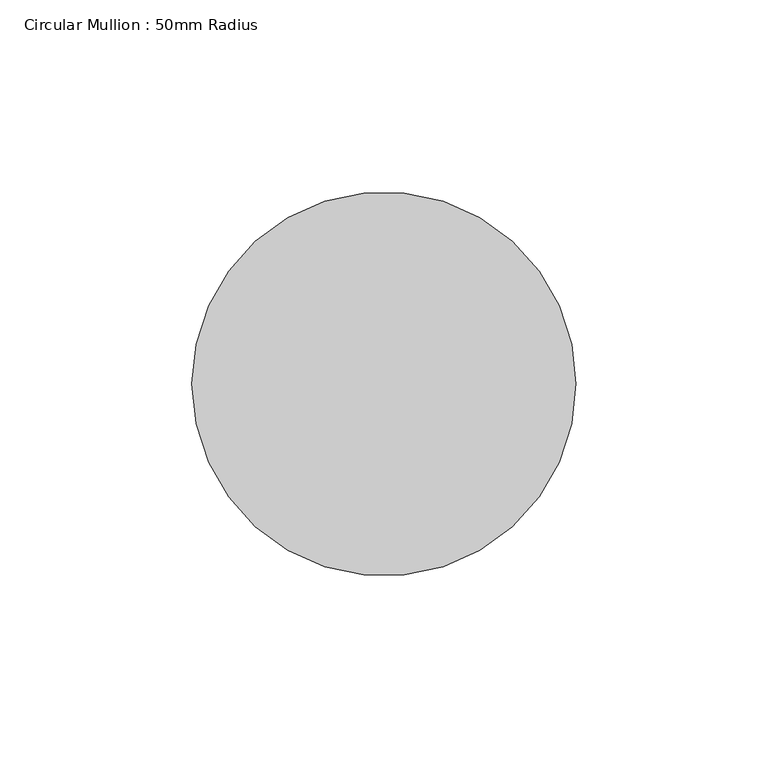
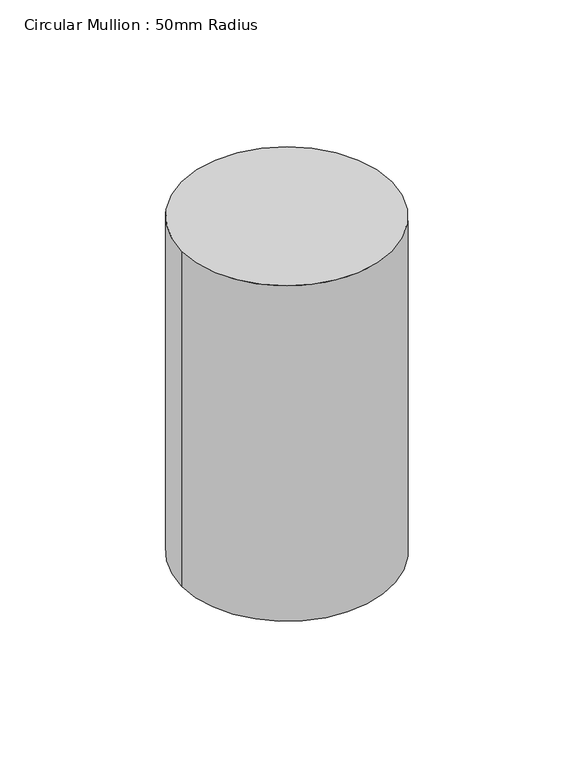
"""IFC4 building model written with IfcOpenShell, lengths in millimetres: member geometry, Circular Mullion : 50mm Radius."""

from ifc_helpers import new_model, si_unit, point, frame, origin, origin_2d, place, context, project, spatial, circle_curve, trimmed, segment, composite_curve, outline, extrude, source, transform, mapped, element, save


def circular_mullion_50mm_radius_9a7782ce(model_context):
    return source(origin(), model_context, "Body", "SweptSolid", [
        extrude(outline(composite_curve([segment(trimmed(circle_curve(origin_2d(), 50.0), [point((50.0, 0.0))], [point((-50.0, 0.0))], False, "CARTESIAN"), True, "CONTINUOUS"), segment(trimmed(circle_curve(origin_2d(), 50.0), [point((-50.0, 0.0))], [point((50.0, 0.0))], False, "CARTESIAN"), True, "CONTINUOUS")], self_intersect=False)), frame((0.0, 0.0, -168.6719709), z_axis=(0.0, 0.0, 1.0), x_axis=(1.0, 0.0, 0.0)), (0.0, 0.0, 1.0), 168.6719709),
    ])


if __name__ == "__main__":
    model = new_model("IFC4")
    model_context = context("Model", 3, world=origin())
    ifc_project = project(units=[si_unit("LENGTHUNIT", "METRE", prefix="MILLI")], contexts=[model_context])
    site = spatial("IfcSite", under=ifc_project)
    building = spatial("IfcBuilding", under=site)
    placement = place(None, origin())
    circular_mullion_50mm_radius_shape = circular_mullion_50mm_radius_9a7782ce(model_context)
    element("IfcMember", 1, ObjectType="Circular Mullion : 50mm Radius", at=placement, inside=building, context=model_context, shape_type="MappedRepresentation", body=[
        mapped(circular_mullion_50mm_radius_shape, transform((0.0, 0.0, 0.0), x_axis=(1.0, 0.0, 0.0), y_axis=(0.0, 1.0, 0.0), z_axis=(0.0, 0.0, 1.0))),
    ])
    save(model, "model.ifc")

# Revit data of these elements
# Type "Circular Mullion : 50mm Radius"
#   built-in parameter 1007350 = 0.164042 (stored number, unit not read)
# Element 1 (IfcMember, "Circular Mullion : 50mm Radius")
#   Materials on its faces: "Aluminium"
# Materials
#   "Aluminium": class "Metal", colour RGB 247 247 247, transparency 0, Description = "Aluminium 6061", Cost = 0
